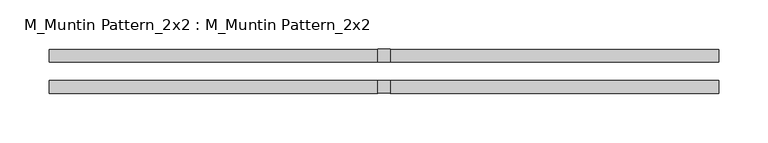
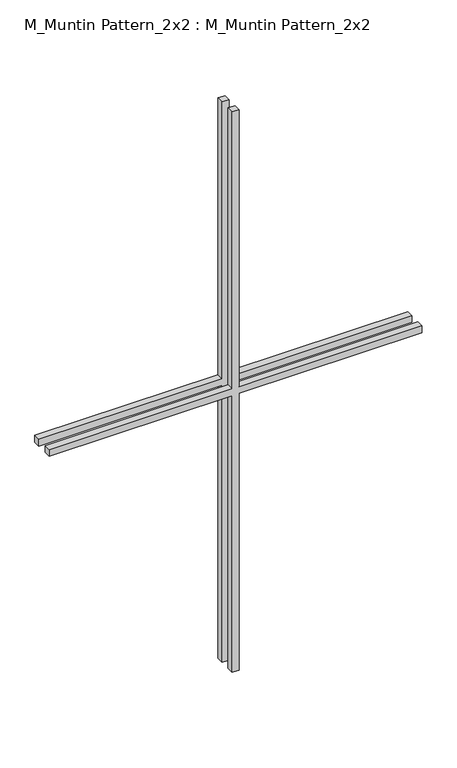
"""IFC4 building model written with IfcOpenShell, lengths in millimetres: proxy geometry, M_Muntin Pattern_2x2 : M_Muntin Pattern_2x2."""

from ifc_helpers import new_model, si_unit, frame, origin, place, context, project, spatial, polyline, outline, extrude, source, transform, mapped, element, save


def m_muntin_pattern_2x2_m_muntin_pattern_2x2_3179e719(model_context):
    return source(origin(), model_context, "Body", "SweptSolid", [
        extrude(outline(polyline([(542.925, -6.35), (542.925, -338.1375), (530.225, -338.1375), (530.225, -6.35), (0.0, -6.35), (0.0, 6.35), (530.225, 6.35), (530.225, 338.1375), (542.925, 338.1375), (542.925, 6.35), (1073.15, 6.35), (1073.15, -6.35), (542.925, -6.35)])), frame((0.0, 9.525, 0.0), z_axis=(0.0, 1.0, 0.0), x_axis=(0.0, 0.0, 1.0)), (0.0, 0.0, 1.0), 12.7),
        extrude(outline(polyline([(542.925, -6.35), (542.925, -338.1375), (530.225, -338.1375), (530.225, -6.35), (0.0, -6.35), (0.0, 6.35), (530.225, 6.35), (530.225, 338.1375), (542.925, 338.1375), (542.925, 6.35), (1073.15, 6.35), (1073.15, -6.35), (542.925, -6.35)])), frame((0.0, -22.225, 0.0), z_axis=(0.0, 1.0, 0.0), x_axis=(0.0, 0.0, 1.0)), (0.0, 0.0, 1.0), 12.7),
    ])


if __name__ == "__main__":
    model = new_model("IFC4")
    model_context = context("Model", 3, world=origin())
    ifc_project = project(units=[si_unit("LENGTHUNIT", "METRE", prefix="MILLI")], contexts=[model_context])
    site = spatial("IfcSite", under=ifc_project)
    building = spatial("IfcBuilding", under=site)
    placement = place(None, origin())
    m_muntin_pattern_2x2_m_muntin_pattern_2x2_shape = m_muntin_pattern_2x2_m_muntin_pattern_2x2_3179e719(model_context)
    element("IfcBuildingElementProxy", 1, Name="M_Muntin Pattern_2x2 : M_Muntin Pattern_2x2", ObjectType="M_Muntin Pattern_2x2 : M_Muntin Pattern_2x2", at=placement, inside=building, context=model_context, shape_type="MappedRepresentation", body=[
        mapped(m_muntin_pattern_2x2_m_muntin_pattern_2x2_shape, transform((0.0, 0.0, 0.0), x_axis=(1.0, 0.0, 0.0), y_axis=(0.0, 1.0, 0.0), z_axis=(0.0, 0.0, 1.0))),
    ])
    save(model, "model.ifc")

# Revit data of these elements
# Type "M_Muntin Pattern_2x2 : M_Muntin Pattern_2x2"
#   Width [instance default] = 3' - 11.24409"
#   Thickness = 0' - 0 1/2"
#   Height [instance default] = 3' - 11.24409"
#   Distance = 0' - 0 3/4"
#   Interior Material [instance default] = none
#   Exterior Material [instance default] = none
#   Default Elevation = 0
# Element 1 (IfcBuildingElementProxy, "M_Muntin Pattern_2x2 : M_Muntin Pattern_2x2")
#   Width = 2' - 2 5/8"
#   Height = 3' - 6 1/4"
#   Interior Material = Wood - Stained
#   Exterior Material = Clad - White
#   Materials on its faces: "Clad - White", "Wood - Stained"
# Materials
#   "Clad - White": class "Wood", colour RGB 242 242 238, transparency 0, Cost = 0
#   "Wood - Stained": class "Wood", colour RGB 224 178 126, transparency 0, Cost = 0
